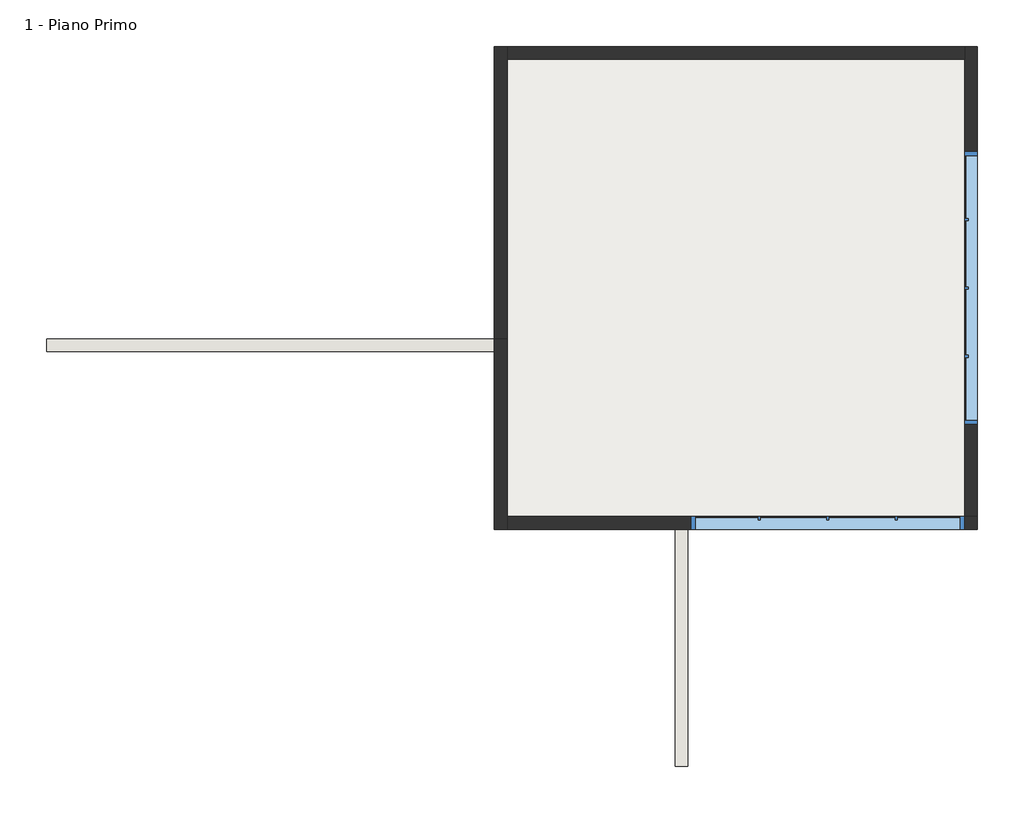
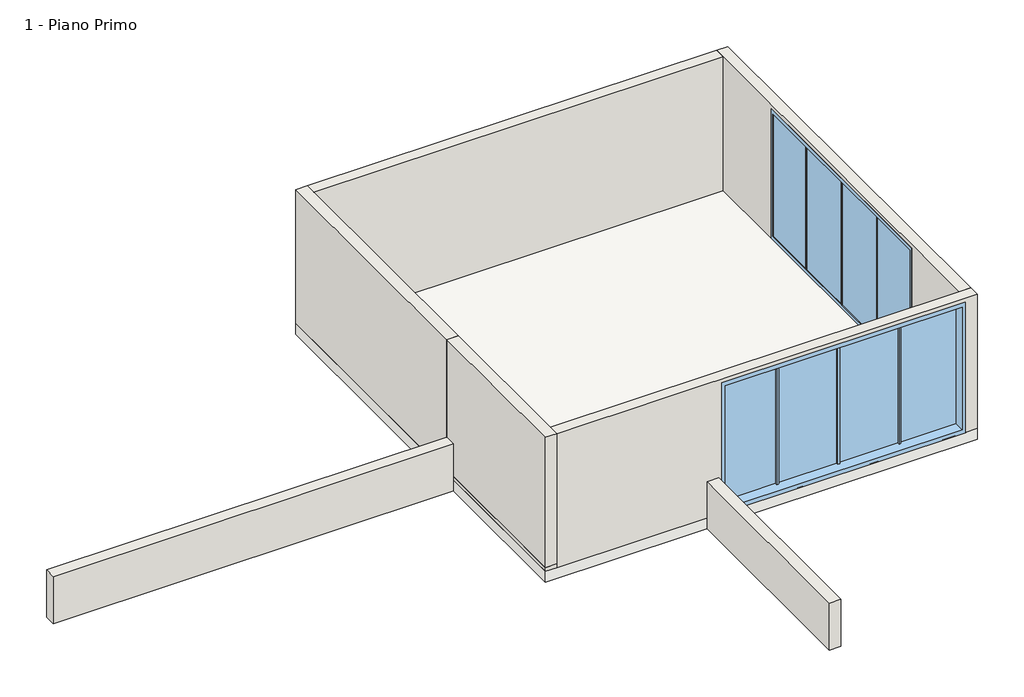
# One storey: 8 walls, 2 windows, 1 slab.
"""IFC4 building model written with IfcOpenShell, lengths in millimetres."""

import ifcopenshell
import ifcopenshell.guid

model = None  # the IFC model being written
_history = None  # IfcOwnerHistory: only IFC2X3 demands one
_inside = {}  # id of a spatial element -> (the spatial element, [elements in it])
_under = {}  # id of a project, library or spatial element -> (it, [spatial elements below it])
_declared = {}  # id of a project -> (the project, [libraries it declares])
_typed = {}  # id of a type object -> (the type object, [elements of that type])
_made_of = {}  # id of a material, layer set ... -> (it, [elements and type objects made of it])


def new_model(schema):
    """Start an empty IFC model of exactly this schema.

    Asked for "IFC4X3", IfcOpenShell would pick the latest addendum, in which some entities
    have other attributes; the version numbers below select the first issue.
    IFC2X3 requires an IfcOwnerHistory on every rooted entity: one is made here for all.
    """
    global model, _history
    if schema == "IFC4X3":
        model = ifcopenshell.file(schema_version=(4, 3, 0, 0))
    else:
        model = ifcopenshell.file(schema=schema)
    _inside.clear()
    _under.clear()
    _declared.clear()
    _typed.clear()
    _made_of.clear()
    _history = None
    if model.schema == "IFC2X3":
        org = make("IfcOrganization", Name="unknown")
        user = make(
            "IfcPersonAndOrganization",
            ThePerson=make("IfcPerson", FamilyName="unknown"),
            TheOrganization=org,
        )
        app = make(
            "IfcApplication",
            ApplicationDeveloper=org,
            Version="unknown",
            ApplicationFullName="unknown",
            ApplicationIdentifier="unknown",
        )
        _history = make(
            "IfcOwnerHistory",
            OwningUser=user,
            OwningApplication=app,
            ChangeAction="ADDED",
            CreationDate=0,
        )
    return model


def make(cls, **values):
    """One entity of the class cls with the attributes given. An attribute that is None is left unset."""
    return model.create_entity(
        cls, **{name: value for name, value in values.items() if value is not None}
    )


def rooted(cls, **values):
    """An entity with a GlobalId (a new one), such as an element, a storey or a relation."""
    return make(cls, GlobalId=ifcopenshell.guid.new(), OwnerHistory=_history, **values)


def si_unit(unit_type, name, prefix=None):
    """IfcSIUnit, for example si_unit("LENGTHUNIT", "METRE", prefix="MILLI")."""
    return make("IfcSIUnit", UnitType=unit_type, Prefix=prefix, Name=name)


def assignment(units):
    """IfcUnitAssignment: the units of a project."""
    return None if units is None else make("IfcUnitAssignment", Units=units)


def point(xyz):
    """IfcCartesianPoint."""
    return None if xyz is None else make("IfcCartesianPoint", Coordinates=xyz)


def direction(xyz):
    """IfcDirection."""
    return None if xyz is None else make("IfcDirection", DirectionRatios=xyz)


def frame(location, z_axis=None, x_axis=None):
    """IfcAxis2Placement3D, a coordinate frame: its origin and axes. An axis left out is left unset."""
    return make(
        "IfcAxis2Placement3D",
        Location=point(location),
        Axis=direction(z_axis),
        RefDirection=direction(x_axis),
    )


def origin():
    """The frame at (0, 0, 0) with its axes left unset."""
    return frame((0.0, 0.0, 0.0))


def place(relative_to, where):
    """IfcLocalPlacement: puts the frame where relative to a parent placement (None: the world)."""
    return make(
        "IfcLocalPlacement", PlacementRelTo=relative_to, RelativePlacement=where
    )


def context(
    kind, dimensions, precision=None, world=None, true_north=None, identifier=None
):
    """IfcGeometricRepresentationContext, for example the 3D "Model" context."""
    return make(
        "IfcGeometricRepresentationContext",
        ContextIdentifier=identifier,
        ContextType=kind,
        CoordinateSpaceDimension=dimensions,
        Precision=precision,
        WorldCoordinateSystem=world,
        TrueNorth=true_north,
    )


def project(units=None, contexts=None):
    """IfcProject with its units and contexts."""
    return rooted(
        "IfcProject",
        Name="project",
        RepresentationContexts=contexts,
        UnitsInContext=assignment(units),
    )


def spatial(cls, under=None, at=None, **own):
    """A site, building, storey or space (cls), placed at a placement, below another one or the project."""
    s = rooted(cls, ObjectPlacement=at, **own)
    if under is not None:
        _under.setdefault(under.id(), (under, []))[1].append(s)
    return s


def polyline(points):
    """IfcPolyline through the points."""
    return make("IfcPolyline", Points=[point(p) for p in points])


def outline(outer, holes=None, kind="AREA"):
    """IfcArbitraryClosedProfileDef: a profile drawn as a closed curve; with holes, ...WithVoids."""
    if holes is None:
        return make("IfcArbitraryClosedProfileDef", ProfileType=kind, OuterCurve=outer)
    return make(
        "IfcArbitraryProfileDefWithVoids",
        ProfileType=kind,
        OuterCurve=outer,
        InnerCurves=holes,
    )


def extrude(swept, where, along, depth):
    """IfcExtrudedAreaSolid: the profile swept, set in the frame where, extruded along a direction by depth."""
    return make(
        "IfcExtrudedAreaSolid",
        SweptArea=swept,
        Position=where,
        ExtrudedDirection=direction(along),
        Depth=depth,
    )


def faces_of(points, faces, orient=None, outer=None):
    """IfcFace entities. A face is a list of loops; a loop is a list of indices into points, from 0.

    orient and outer hold one flag for each loop. By default every Orientation is true, the
    first loop of a face is its IfcFaceOuterBound and the others are IfcFaceBound.
    """
    made = []
    for i, loops in enumerate(faces):
        bounds = []
        for j, loop in enumerate(loops):
            is_outer = j == 0 if outer is None else outer[i][j]
            bounds.append(
                make(
                    "IfcFaceOuterBound" if is_outer else "IfcFaceBound",
                    Bound=make("IfcPolyLoop", Polygon=[points[k] for k in loop]),
                    Orientation=True if orient is None else orient[i][j],
                )
            )
        made.append(make("IfcFace", Bounds=bounds))
    return made


def faceted_brep(points, faces, orient=None, outer=None, voids=None):
    """IfcFacetedBrep: a solid bounded by flat faces; with voids (closed shells), ...WithVoids."""
    shared = [point(p) for p in points]
    hull = make("IfcClosedShell", CfsFaces=faces_of(shared, faces, orient, outer))
    if voids is None:
        return make("IfcFacetedBrep", Outer=hull)
    return make(
        "IfcFacetedBrepWithVoids",
        Outer=hull,
        Voids=[
            make(cls, CfsFaces=faces_of(shared, fs, o, b)) for cls, fs, o, b in voids
        ],
    )


def shape(context_of_items, identifier, shape_type, items):
    """IfcShapeRepresentation: the items that make up one representation, for example the "Body"."""
    return make(
        "IfcShapeRepresentation",
        ContextOfItems=context_of_items,
        RepresentationIdentifier=identifier,
        RepresentationType=shape_type,
        Items=items,
    )


def source(mapping_origin, context_of_items, identifier, shape_type, items):
    """IfcRepresentationMap: a shape defined once, which mapped items show again and again."""
    return make(
        "IfcRepresentationMap",
        MappingOrigin=mapping_origin,
        MappedRepresentation=shape(context_of_items, identifier, shape_type, items),
    )


def transform(
    local_origin,
    x_axis=None,
    y_axis=None,
    z_axis=None,
    scale=None,
    scale2=None,
    scale3=None,
    uniform=True,
):
    """IfcCartesianTransformationOperator3D, or its non-uniform kind. x_axis, y_axis, z_axis: its Axis1, 2, 3."""
    if uniform:
        return make(
            "IfcCartesianTransformationOperator3D",
            Axis1=direction(x_axis),
            Axis2=direction(y_axis),
            LocalOrigin=point(local_origin),
            Scale=scale,
            Axis3=direction(z_axis),
        )
    return make(
        "IfcCartesianTransformationOperator3DnonUniform",
        Axis1=direction(x_axis),
        Axis2=direction(y_axis),
        LocalOrigin=point(local_origin),
        Scale=scale,
        Axis3=direction(z_axis),
        Scale2=scale2,
        Scale3=scale3,
    )


def mapped(mapping_source, mapping_target):
    """IfcMappedItem: shows the shape of a source again, moved by a transform."""
    return make(
        "IfcMappedItem", MappingSource=mapping_source, MappingTarget=mapping_target
    )


def made_of(thing, what):
    """Note that an element or type object is made of a material, layer set ...; save() writes the relation."""
    if what is not None:
        _made_of.setdefault(what.id(), (what, []))[1].append(thing)
    return thing


def element(
    cls,
    number,
    at=None,
    inside=None,
    cuts=None,
    type_object=None,
    material=None,
    context=None,
    identifier="Body",
    shape_type=None,
    held_by="IfcProductDefinitionShape",
    body=None,
    shapes=None,
    **own,
):
    """One element of the class cls, such as IfcWall. Its Tag is "e" and its number.

    at: its placement. inside: the storey or other place that contains it. cuts: it is an
    opening in that element (IfcRelVoidsElement). A single representation is given by context,
    identifier, shape_type and body (its items); several are given by shapes. held_by: the class
    of the entity that holds the representations. save() writes the other relations.
    """
    e = rooted(cls, Tag="e%d" % number, ObjectPlacement=at, **own)
    if body is not None:
        shapes = [shape(context, identifier, shape_type, body)]
    if shapes is not None:
        e.Representation = make(held_by, Representations=shapes)
    if inside is not None:
        _inside.setdefault(inside.id(), (inside, []))[1].append(e)
    if cuts is not None:
        rooted(
            "IfcRelVoidsElement", RelatingBuildingElement=cuts, RelatedOpeningElement=e
        )
    if type_object is not None:
        _typed.setdefault(type_object.id(), (type_object, []))[1].append(e)
    return made_of(e, material)


def aggregate(whole, parts):
    """IfcRelAggregates: a whole, such as a stair, and the parts it consists of."""
    return rooted("IfcRelAggregates", RelatingObject=whole, RelatedObjects=parts)


def save(model, path):
    """Write the relations noted so far, then the file.

    IfcRelAggregates (storeys below a building ...), IfcRelContainedInSpatialStructure (elements
    in a storey), IfcRelDefinesByType, IfcRelAssociatesMaterial and IfcRelDeclares: one each for
    every whole, place, type object, material and project.
    """
    for whole, parts in _under.values():
        aggregate(whole, parts)
    for where, things in _inside.values():
        rooted(
            "IfcRelContainedInSpatialStructure",
            RelatedElements=things,
            RelatingStructure=where,
        )
    for kind, things in _typed.values():
        rooted("IfcRelDefinesByType", RelatedObjects=things, RelatingType=kind)
    for what, things in _made_of.values():
        rooted("IfcRelAssociatesMaterial", RelatedObjects=things, RelatingMaterial=what)
    for by, libraries in _declared.values():
        rooted("IfcRelDeclares", RelatingContext=by, RelatedDefinitions=libraries)
    model.write(path)


def window_8667a62f(model_context):
    return source(origin(), model_context, "Body", "SolidModel", [
        faceted_brep([(-3255.5, 149.7451428, 3700.0), (3144.5, 149.7451428, 3700.0), (3144.5, 149.7451428, 80.0), (-3255.5, 149.7451428, 80.0), (-3155.5, 149.7451428, 3580.0), (-3155.5, 149.7451428, 200.0), (-1680.2592993, 149.7451428, 200.0), (-1680.2592993, 149.7451428, 3580.0), (-1630.5, 149.7451428, 200.0), (-80.5, 149.7451428, 200.0), (-80.5, 149.7451428, 3580.0), (-1630.5, 149.7451428, 3580.0), (1519.5, 149.7451428, 200.0), (1519.5, 149.7451428, 3580.0), (-30.5, 149.7451428, 3580.0), (-30.5, 149.7451428, 200.0), (1569.5, 149.7451428, 3580.0), (1569.5, 149.7451428, 200.0), (3044.5, 149.7451428, 200.0), (3044.5, 149.7451428, 3580.0), (-3155.5, -150.2548572, 3580.0), (-3155.5, -150.2548572, 200.0), (3044.5, -150.2548572, 200.0), (1569.5, 67.6275467, 200.0), (1519.5, 67.6275467, 200.0), (-30.5, 67.6275467, 200.0), (-80.5, 67.6275467, 200.0), (-1630.5, 67.6275467, 200.0), (-1680.2592993, 67.6275467, 200.0), (-1680.2592993, 67.6275467, 3580.0), (3144.5, -150.2548572, 3700.0), (3144.5, -150.2548572, 80.0), (-3255.5, -150.2548572, 80.0), (-3255.5, -150.2548572, 3700.0), (-80.5, 67.6275467, 3580.0), (-1630.5, 67.6275467, 3580.0), (1519.5, 67.6275467, 3580.0), (-30.5, 67.6275467, 3580.0), (1569.5, 67.6275467, 3580.0), (3044.5, -150.2548572, 3580.0)], [[[0, 1, 2, 3], [4, 5, 6, 7], [8, 9, 10, 11], [12, 13, 14, 15], [16, 17, 18, 19]], [[20, 21, 5, 4]], [[21, 22, 18, 17, 23, 24, 12, 15, 25, 26, 9, 8, 27, 28, 6, 5]], [[7, 6, 28, 29]], [[30, 31, 2, 1]], [[31, 32, 3, 2]], [[32, 33, 0, 3]], [[10, 9, 26, 34]], [[8, 11, 35, 27]], [[13, 12, 24, 36]], [[15, 14, 37, 25]], [[17, 16, 38, 23]], [[22, 39, 19, 18]], [[36, 24, 23, 38]], [[33, 32, 31, 30], [20, 39, 22, 21]], [[34, 26, 25, 37]], [[29, 28, 27, 35]], [[33, 30, 1, 0]], [[39, 20, 4, 7, 29, 35, 11, 10, 34, 37, 14, 13, 36, 38, 16, 19]]]),
        extrude(outline(polyline([(3044.5, 124.7451428), (1569.5, 124.7451428), (1569.5, 134.7451428), (3044.5, 134.7451428), (3044.5, 124.7451428)])), frame((0.0, 0.0, 200.0), z_axis=(0.0, 0.0, 1.0), x_axis=(1.0, 0.0, 0.0)), (0.0, 0.0, 1.0), 3380.0),
        extrude(outline(polyline([(1519.5, 124.7451428), (-30.5, 124.7451428), (-30.5, 134.7451428), (1519.5, 134.7451428), (1519.5, 124.7451428)])), frame((0.0, 0.0, 200.0), z_axis=(0.0, 0.0, 1.0), x_axis=(1.0, 0.0, 0.0)), (0.0, 0.0, 1.0), 3380.0),
        extrude(outline(polyline([(-80.5, 124.7451428), (-1630.5, 124.7451428), (-1630.5, 134.7451428), (-80.5, 134.7451428), (-80.5, 124.7451428)])), frame((0.0, 0.0, 200.0), z_axis=(0.0, 0.0, 1.0), x_axis=(1.0, 0.0, 0.0)), (0.0, 0.0, 1.0), 3380.0),
        extrude(outline(polyline([(-1680.2592993, 124.7451428), (-3155.5, 124.7451428), (-3155.5, 134.7451428), (-1680.2592993, 134.7451428), (-1680.2592993, 124.7451428)])), frame((0.0, 0.0, 200.0), z_axis=(0.0, 0.0, 1.0), x_axis=(1.0, 0.0, 0.0)), (0.0, 0.0, 1.0), 3380.0),
    ])


model = new_model("IFC4")

# Units and contexts
model_context = context("Model", 3, world=origin())
ifc_project = project(units=[si_unit("LENGTHUNIT", "METRE", prefix="MILLI")], contexts=[model_context])

# Site, building, storey
site = spatial("IfcSite", under=ifc_project)
building = spatial("IfcBuilding", under=site)
storey = spatial("IfcBuildingStorey", under=building, Name="1 - Piano Primo", Elevation=4000.0)

# Slab
placement = place(None, origin())
element("IfcSlab", 1, ObjectType="Latero Cementizio - 30 cm", at=placement, inside=storey, context=model_context, shape_type="SweptSolid", body=[
    extrude(outline(polyline([(13577.4891128, 14171.5492236), (13577.4891128, 2871.5492236), (2277.4891128, 2871.5492236), (2277.4891128, 14171.5492236), (13577.4891128, 14171.5492236)])), frame((0.0, 0.0, 3700.0), z_axis=(0.0, 0.0, 1.0), x_axis=(1.0, 0.0, 0.0)), (0.0, 0.0, 1.0), 300.0),
])

# Walls
element("IfcWall", 2, ObjectType="Generico - 30 cm", at=placement, inside=storey, context=model_context, shape_type="Brep", body=[
    faceted_brep([(2277.4891128, 14171.5492236, 4000.0), (2277.4891128, 7331.5492236, 4000.0), (2277.4891128, 7331.5492236, 4100.0), (2277.4891128, 7331.5492236, 7700.0), (2277.4891128, 14171.5492236, 7700.0), (2577.4891128, 14171.5492236, 4000.0), (2577.4891128, 14171.5492236, 7700.0), (2577.4891128, 13871.5492236, 7700.0), (2577.4891128, 7331.5492236, 7700.0), (2577.4891128, 7331.5492236, 4100.0), (2577.4891128, 7331.5492236, 4000.0), (2577.4891128, 13871.5492236, 4000.0)], [[[0, 1, 2, 3, 4]], [[5, 6, 7, 8, 9, 10, 11]], [[1, 0, 5, 11, 10]], [[0, 4, 6, 5]], [[1, 10, 9, 8, 3, 2]], [[4, 3, 8, 7, 6]]]),
])
element("IfcWall", 3, ObjectType="Generico - 30 cm", at=placement, inside=storey, context=model_context, shape_type="Brep", body=[
    faceted_brep([(13577.4891128, 2871.5492236, 4000.0), (13577.4891128, 2871.5492236, 7700.0), (2577.4891128, 2871.5492236, 7700.0), (2577.4891128, 2871.5492236, 4100.0), (2577.4891128, 2871.5492236, 4000.0), (6877.4891128, 2871.5492236, 4000.0), (6877.4891128, 2871.5492236, 7600.0), (13277.4891128, 2871.5492236, 7600.0), (13277.4891128, 2871.5492236, 4000.0), (13577.4891128, 3171.5492236, 7700.0), (13577.4891128, 3171.5492236, 4000.0), (13277.4891128, 3171.5492236, 4000.0), (13277.4891128, 3171.5492236, 7600.0), (6877.4891128, 3171.5492236, 7600.0), (6877.4891128, 3171.5492236, 4000.0), (2577.4891128, 3171.5492236, 4000.0), (2577.4891128, 3171.5492236, 7700.0), (13277.4891128, 3171.5492236, 7700.0)], [[[0, 1, 2, 3, 4, 5, 6, 7, 8]], [[9, 10, 11, 12, 13, 14, 15, 16, 17]], [[4, 15, 14, 5]], [[10, 0, 8, 11]], [[1, 0, 10, 9]], [[15, 4, 3, 2, 16]], [[2, 1, 9, 17, 16]], [[13, 6, 5, 14]], [[6, 13, 12, 7]], [[7, 12, 11, 8]]]),
])
element("IfcWall", 4, ObjectType="Generico - 30 cm", at=placement, inside=storey, context=model_context, shape_type="SweptSolid", body=[
    extrude(outline(polyline([(2577.4891128, 14171.5492236), (13277.4891128, 14171.5492236), (13277.4891128, 13871.5492236), (2577.4891128, 13871.5492236), (2577.4891128, 14171.5492236)])), frame((0.0, 0.0, 4000.0), z_axis=(0.0, 0.0, 1.0), x_axis=(1.0, 0.0, 0.0)), (0.0, 0.0, 1.0), 3700.0),
])
element("IfcWall", 5, ObjectType="Generico - 30 cm", at=placement, inside=storey, context=model_context, shape_type="Brep", body=[
    faceted_brep([(2277.4891128, 7331.5492236, 4000.0), (2277.4891128, 2871.5492236, 4000.0), (2277.4891128, 2871.5492236, 4100.0), (2277.4891128, 7331.5492236, 4100.0), (2577.4891128, 7331.5492236, 4000.0), (2577.4891128, 7331.5492236, 4100.0), (2577.4891128, 2871.5492236, 4100.0), (2577.4891128, 2871.5492236, 4000.0), (2577.4891128, 3171.5492236, 4000.0)], [[[0, 1, 2, 3]], [[4, 5, 6, 7, 8]], [[1, 0, 4, 8, 7]], [[3, 2, 6, 5]], [[0, 3, 5, 4]], [[2, 1, 7, 6]]]),
])
element("IfcWall", 6, ObjectType="Generico - 30 cm", at=placement, inside=storey, context=model_context, shape_type="Brep", body=[
    faceted_brep([(2277.4891128, 7331.5492236, 4100.0), (2277.4891128, 2871.5492236, 4100.0), (2277.4891128, 2871.5492236, 7700.0), (2277.4891128, 7331.5492236, 7700.0), (2577.4891128, 7331.5492236, 4100.0), (2577.4891128, 7331.5492236, 7700.0), (2577.4891128, 3171.5492236, 7700.0), (2577.4891128, 2871.5492236, 7700.0), (2577.4891128, 2871.5492236, 4100.0)], [[[0, 1, 2, 3]], [[4, 5, 6, 7, 8]], [[1, 0, 4, 8]], [[0, 3, 5, 4]], [[2, 1, 8, 7]], [[3, 2, 7, 6, 5]]]),
])
element("IfcWall", 7, ObjectType="Generico - 30 cm", at=placement, inside=storey, context=model_context, shape_type="SweptSolid", body=[
    extrude(outline(polyline([(6806.6179856, 2871.5492236), (6806.6179856, -2671.3546615), (6506.6179856, -2671.3546615), (6506.6179856, 2871.5492236), (6806.6179856, 2871.5492236)])), frame((0.0, 0.0, 3700.0), z_axis=(0.0, 0.0, 1.0), x_axis=(1.0, 0.0, 0.0)), (0.0, 0.0, 1.0), 1300.0),
])
element("IfcWall", 8, ObjectType="Generico - 30 cm", at=placement, inside=storey, context=model_context, shape_type="SweptSolid", body=[
    extrude(outline(polyline([(2277.4891128, 7028.6453385), (-8193.3820144, 7028.6453385), (-8193.3820144, 7328.6453385), (2277.4891128, 7328.6453385), (2277.4891128, 7028.6453385)])), frame((0.0, 0.0, 3700.0), z_axis=(0.0, 0.0, 1.0), x_axis=(1.0, 0.0, 0.0)), (0.0, 0.0, 1.0), 1300.0),
])
element("IfcWall", 9, ObjectType="legno", at=placement, inside=storey, context=model_context, shape_type="Brep", body=[
    faceted_brep([(13577.4891128, 3171.5492236, 7700.0), (13577.4891128, 3171.5492236, 4000.0), (13577.4891128, 5321.5492236, 4000.0), (13577.4891128, 5321.5492236, 7600.0), (13577.4891128, 11721.5492236, 7600.0), (13577.4891128, 11721.5492236, 4000.0), (13577.4891128, 14171.5492236, 4000.0), (13577.4891128, 14171.5492236, 7700.0), (13277.4891128, 3171.5492236, 4000.0), (13277.4891128, 3171.5492236, 7600.0), (13277.4891128, 3171.5492236, 7700.0), (13277.4891128, 13871.5492236, 7700.0), (13277.4891128, 14171.5492236, 7700.0), (13277.4891128, 14171.5492236, 4000.0), (13277.4891128, 13871.5492236, 4000.0), (13277.4891128, 11721.5492236, 4000.0), (13277.4891128, 11721.5492236, 7600.0), (13277.4891128, 5321.5492236, 7600.0), (13277.4891128, 5321.5492236, 4000.0)], [[[0, 1, 2, 3, 4, 5, 6, 7]], [[8, 9, 10, 11, 12, 13, 14, 15, 16, 17, 18]], [[1, 8, 18, 2]], [[13, 6, 5, 15, 14]], [[1, 0, 10, 9, 8]], [[7, 6, 13, 12]], [[0, 7, 12, 11, 10]], [[17, 3, 2, 18]], [[3, 17, 16, 4]], [[4, 16, 15, 5]]]),
])

# Windows
window_shape = window_8667a62f(model_context)
element("IfcWindow", 10, ObjectType="Finestra Assemblata : vetrata uffici1", at=placement, inside=storey, context=model_context, shape_type="MappedRepresentation", body=[
    mapped(window_shape, transform((10132.9891128, 3021.8040808, 3900.0), x_axis=(1.0, 0.0, 0.0), y_axis=(0.0, 1.0, 0.0), z_axis=(0.0, 0.0, 1.0))),
])
element("IfcWindow", 11, ObjectType="Finestra Assemblata : vetrata uffici1", at=placement, inside=storey, context=model_context, shape_type="MappedRepresentation", body=[
    mapped(window_shape, transform((13427.2342556, 8577.0492236, 3900.0), x_axis=(0.0, 1.0, 0.0), y_axis=(-1.0, 0.0, 0.0), z_axis=(0.0, 0.0, 1.0))),
])

save(model, "model.ifc")

# Revit data of these elements
# Type "Latero Cementizio - 30 cm"
#   Keynote = "S/3"
#   Function = 0
#   Layers, outside or top first: 0.02 m "Ceramica bianca" (function 4); 0.065 m "Sabbia e Calcestruzzo" (function 2); 0.04 m "Calcestruzzo" (function 1); 0.16 m "Laterizio (2)" (function 1); 0.015 m "Intonaco - Bianco" (function 5)
# Type "Generico - 30 cm"
#   Keynote = "Mb/3"
#   Layers, outside or top first: 0.30 m "Default - Muro" (function 1)
# Type "legno"
#   Keynote = "Mb/3"
#   Layers, outside or top first: 0.01 m "Intonaco - Bianco" (function 1); 0.28 m no material (function 1); 0.01 m "Ciliegia" (function 1)
# Type "Finestra Assemblata : vetrata uffici1"
#   Type Mark = "33"
#   Construction Type Id = "GSP4R"
#   Analytic Construction = "Vetrata singola Pilkington 1/8 in"
#   Visual Light Transmittance = 0.9
#   Solar Heat Gain Coefficient = 0.78
#   Heat Transfer Coefficient (U) = 3.6886 W/(m²·K)
#   MONTANTE = 1.60 m
#   Luce sup = 0.50 m
#   Height = 3.60 m
#   Altezza soglia = 0.10 m
#   Width = 6.40 m
#   Vetro = Default - Vetro
#   Telaio/montante = Metallo - Acciaio inox, levigato
#   Davanzale = Metallo - Acciaio inox, levigato
#   Manufacturer = ""
#   Wall Closure = (empty or 0)
# Element 1 (IfcSlab, "Latero Cementizio - 30 cm")
#   Height Offset From Level = 0.00 m
#   Phase Created = Stato di Progetto
#   Materials on its faces: "Intonaco - Bianco", "Ceramica bianca"
# Elements 2, 4 (IfcWall, "Generico - 30 cm")
#   Top Offset = 0.00 m
#   Base Offset = 0.00 m
#   Unconnected Height = 4.00 m
#   wall height = 4.00 m
#   Phase Created = Stato di Progetto
#   Base Constraint = 1 - Piano Primo
#   Materials on its faces: "Default - Muro"
# Element 3 (IfcWall, "Generico - 30 cm")
#   Top Offset = 0.00 m
#   Base Offset = 0.00 m
#   Unconnected Height = 4.00 m
#   wall height = 4.00 m
#   Phase Created = Stato di Progetto
#   Base Constraint = 1 - Piano Primo
#   Materials on its faces: "Default - Muro", "Ciliegia"
# Element 5 (IfcWall, "Generico - 30 cm")
#   Top Offset = 0.00 m
#   Base Offset = 0.00 m
#   Unconnected Height = 0.10 m
#   wall height = 0.10 m
#   Phase Created = Stato di Progetto
#   Base Constraint = 1 - Piano Primo
#   Materials on its faces: "Default - Muro"
# Element 6 (IfcWall, "Generico - 30 cm")
#   built-in parameter 1001111 = 0.10 m
#   Top Offset = 0.00 m
#   Base Offset = 0.10 m
#   Unconnected Height = 3.90 m
#   wall height = 3.90 m
#   Phase Created = Stato di Progetto
#   Base Constraint = 1 - Piano Primo
#   Materials on its faces: "Default - Muro"
# Elements 7, 8 (IfcWall, "Generico - 30 cm")
#   built-in parameter 1001111 = -0.30 m
#   Top Offset = 0.00 m
#   Base Offset = -0.30 m
#   Unconnected Height = 1.30 m
#   wall height = 1.30 m
#   Phase Created = Stato di Progetto
#   Base Constraint = 1 - Piano Primo
#   Materials on its faces: "Default - Muro"
# Element 9 (IfcWall, "legno")
#   Top Offset = 0.00 m
#   Base Offset = 0.00 m
#   Unconnected Height = 4.00 m
#   wall height = 4.00 m
#   Phase Created = Stato di Progetto
#   Base Constraint = 1 - Piano Primo
#   Materials on its faces: "Default - Calcestruzzo", "Ciliegia", "Intonaco - Bianco", "Default - Muro"
# Element 10 (IfcWindow, "Finestra Assemblata : vetrata uffici1")
#   Mark = "5"
#   Phase Created = Stato di Progetto
#   Materials on its faces: "Metallo - Acciaio inox, levigato", "Default - Vetro"
# Element 11 (IfcWindow, "Finestra Assemblata : vetrata uffici1")
#   Mark = "2"
#   Phase Created = Stato di Progetto
#   Materials on its faces: "Metallo - Acciaio inox, levigato", "Default - Vetro"
# Materials
#   "Ceramica bianca": class "Ceramica", colour RGB 210 210 210, transparency 0, Description = "Finitura interna - Piastrelle di ceramica incollate", Cost = 0
#   "Sabbia e Calcestruzzo": class "Calcestruzzo", colour RGB 127 127 127, transparency 0, Description = "Magrone - Sabbia e cemento", Cost = 0
#   "Calcestruzzo": class "Calcestruzzo", colour RGB 192 192 192, transparency 0, Description = "Calcestruzzo - Cemento Portland", Cost = 0
#   "Laterizio (2)": class "Mattone", colour RGB 255 128 64, transparency 0, Description = "Pignatta h 16 cm", Cost = 0
#   "Intonaco - Bianco": class "Intonaco", colour RGB 249 249 249, transparency 0, Description = "Verniciatura", Cost = 0
#   "Default - Muro": class "Varie", colour RGB 127 127 127, transparency 0, Cost = 0
#   "Ciliegia": class "Legno", colour RGB 226 177 128, transparency 0, Description = "Ciliegio tardivo", Cost = 0
#   "Default - Vetro": class "Vetro", colour RGB 208 208 208, transparency 0.7, Cost = 0
#   "Metallo - Acciaio inox, levigato": class "Metallo", colour RGB 236 239 239, transparency 0, Cost = 0
#   "Default - Calcestruzzo": class "Calcestruzzo", colour RGB 192 192 192, transparency 0, Description = "Calcestruzzo", Cost = 0
